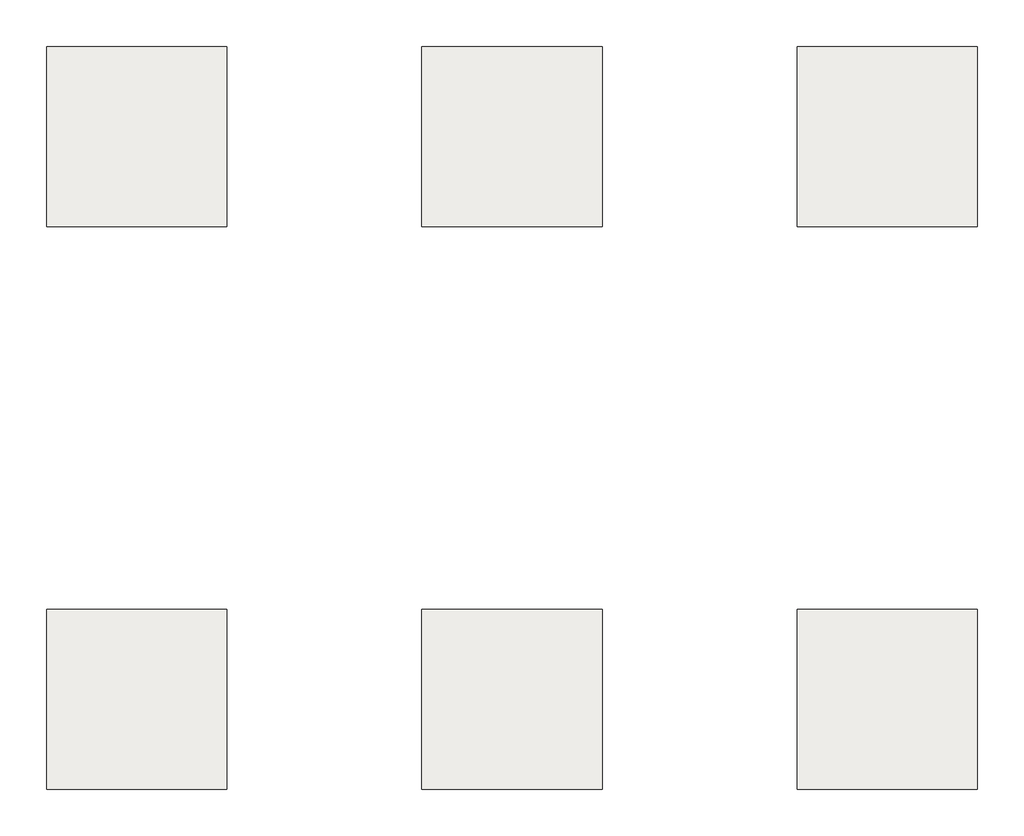
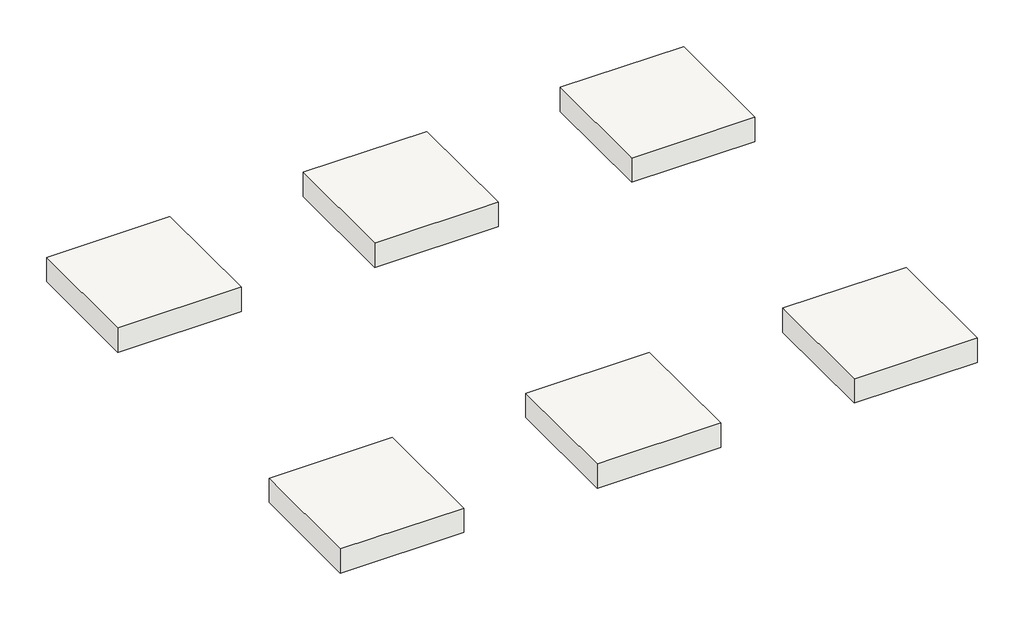
# Not in any storey: 6 slabs.
"""IFC4 building model written with IfcOpenShell, lengths in millimetres."""

import ifcopenshell
import ifcopenshell.guid

model = None  # the IFC model being written
_history = None  # IfcOwnerHistory: only IFC2X3 demands one
_inside = {}  # id of a spatial element -> (the spatial element, [elements in it])
_under = {}  # id of a project, library or spatial element -> (it, [spatial elements below it])
_declared = {}  # id of a project -> (the project, [libraries it declares])
_typed = {}  # id of a type object -> (the type object, [elements of that type])
_made_of = {}  # id of a material, layer set ... -> (it, [elements and type objects made of it])


def new_model(schema):
    """Start an empty IFC model of exactly this schema.

    Asked for "IFC4X3", IfcOpenShell would pick the latest addendum, in which some entities
    have other attributes; the version numbers below select the first issue.
    IFC2X3 requires an IfcOwnerHistory on every rooted entity: one is made here for all.
    """
    global model, _history
    if schema == "IFC4X3":
        model = ifcopenshell.file(schema_version=(4, 3, 0, 0))
    else:
        model = ifcopenshell.file(schema=schema)
    _inside.clear()
    _under.clear()
    _declared.clear()
    _typed.clear()
    _made_of.clear()
    _history = None
    if model.schema == "IFC2X3":
        org = make("IfcOrganization", Name="unknown")
        user = make(
            "IfcPersonAndOrganization",
            ThePerson=make("IfcPerson", FamilyName="unknown"),
            TheOrganization=org,
        )
        app = make(
            "IfcApplication",
            ApplicationDeveloper=org,
            Version="unknown",
            ApplicationFullName="unknown",
            ApplicationIdentifier="unknown",
        )
        _history = make(
            "IfcOwnerHistory",
            OwningUser=user,
            OwningApplication=app,
            ChangeAction="ADDED",
            CreationDate=0,
        )
    return model


def make(cls, **values):
    """One entity of the class cls with the attributes given. An attribute that is None is left unset."""
    return model.create_entity(
        cls, **{name: value for name, value in values.items() if value is not None}
    )


def rooted(cls, **values):
    """An entity with a GlobalId (a new one), such as an element, a storey or a relation."""
    return make(cls, GlobalId=ifcopenshell.guid.new(), OwnerHistory=_history, **values)


def si_unit(unit_type, name, prefix=None):
    """IfcSIUnit, for example si_unit("LENGTHUNIT", "METRE", prefix="MILLI")."""
    return make("IfcSIUnit", UnitType=unit_type, Prefix=prefix, Name=name)


def assignment(units):
    """IfcUnitAssignment: the units of a project."""
    return None if units is None else make("IfcUnitAssignment", Units=units)


def point(xyz):
    """IfcCartesianPoint."""
    return None if xyz is None else make("IfcCartesianPoint", Coordinates=xyz)


def direction(xyz):
    """IfcDirection."""
    return None if xyz is None else make("IfcDirection", DirectionRatios=xyz)


def frame(location, z_axis=None, x_axis=None):
    """IfcAxis2Placement3D, a coordinate frame: its origin and axes. An axis left out is left unset."""
    return make(
        "IfcAxis2Placement3D",
        Location=point(location),
        Axis=direction(z_axis),
        RefDirection=direction(x_axis),
    )


def origin():
    """The frame at (0, 0, 0) with its axes left unset."""
    return frame((0.0, 0.0, 0.0))


def place(relative_to, where):
    """IfcLocalPlacement: puts the frame where relative to a parent placement (None: the world)."""
    return make(
        "IfcLocalPlacement", PlacementRelTo=relative_to, RelativePlacement=where
    )


def context(
    kind, dimensions, precision=None, world=None, true_north=None, identifier=None
):
    """IfcGeometricRepresentationContext, for example the 3D "Model" context."""
    return make(
        "IfcGeometricRepresentationContext",
        ContextIdentifier=identifier,
        ContextType=kind,
        CoordinateSpaceDimension=dimensions,
        Precision=precision,
        WorldCoordinateSystem=world,
        TrueNorth=true_north,
    )


def project(units=None, contexts=None):
    """IfcProject with its units and contexts."""
    return rooted(
        "IfcProject",
        Name="project",
        RepresentationContexts=contexts,
        UnitsInContext=assignment(units),
    )


def spatial(cls, under=None, at=None, **own):
    """A site, building, storey or space (cls), placed at a placement, below another one or the project."""
    s = rooted(cls, ObjectPlacement=at, **own)
    if under is not None:
        _under.setdefault(under.id(), (under, []))[1].append(s)
    return s


def polyline(points):
    """IfcPolyline through the points."""
    return make("IfcPolyline", Points=[point(p) for p in points])


def outline(outer, holes=None, kind="AREA"):
    """IfcArbitraryClosedProfileDef: a profile drawn as a closed curve; with holes, ...WithVoids."""
    if holes is None:
        return make("IfcArbitraryClosedProfileDef", ProfileType=kind, OuterCurve=outer)
    return make(
        "IfcArbitraryProfileDefWithVoids",
        ProfileType=kind,
        OuterCurve=outer,
        InnerCurves=holes,
    )


def extrude(swept, where, along, depth):
    """IfcExtrudedAreaSolid: the profile swept, set in the frame where, extruded along a direction by depth."""
    return make(
        "IfcExtrudedAreaSolid",
        SweptArea=swept,
        Position=where,
        ExtrudedDirection=direction(along),
        Depth=depth,
    )


def shape(context_of_items, identifier, shape_type, items):
    """IfcShapeRepresentation: the items that make up one representation, for example the "Body"."""
    return make(
        "IfcShapeRepresentation",
        ContextOfItems=context_of_items,
        RepresentationIdentifier=identifier,
        RepresentationType=shape_type,
        Items=items,
    )


def source(mapping_origin, context_of_items, identifier, shape_type, items):
    """IfcRepresentationMap: a shape defined once, which mapped items show again and again."""
    return make(
        "IfcRepresentationMap",
        MappingOrigin=mapping_origin,
        MappedRepresentation=shape(context_of_items, identifier, shape_type, items),
    )


def transform(
    local_origin,
    x_axis=None,
    y_axis=None,
    z_axis=None,
    scale=None,
    scale2=None,
    scale3=None,
    uniform=True,
):
    """IfcCartesianTransformationOperator3D, or its non-uniform kind. x_axis, y_axis, z_axis: its Axis1, 2, 3."""
    if uniform:
        return make(
            "IfcCartesianTransformationOperator3D",
            Axis1=direction(x_axis),
            Axis2=direction(y_axis),
            LocalOrigin=point(local_origin),
            Scale=scale,
            Axis3=direction(z_axis),
        )
    return make(
        "IfcCartesianTransformationOperator3DnonUniform",
        Axis1=direction(x_axis),
        Axis2=direction(y_axis),
        LocalOrigin=point(local_origin),
        Scale=scale,
        Axis3=direction(z_axis),
        Scale2=scale2,
        Scale3=scale3,
    )


def mapped(mapping_source, mapping_target):
    """IfcMappedItem: shows the shape of a source again, moved by a transform."""
    return make(
        "IfcMappedItem", MappingSource=mapping_source, MappingTarget=mapping_target
    )


def made_of(thing, what):
    """Note that an element or type object is made of a material, layer set ...; save() writes the relation."""
    if what is not None:
        _made_of.setdefault(what.id(), (what, []))[1].append(thing)
    return thing


def element(
    cls,
    number,
    at=None,
    inside=None,
    cuts=None,
    type_object=None,
    material=None,
    context=None,
    identifier="Body",
    shape_type=None,
    held_by="IfcProductDefinitionShape",
    body=None,
    shapes=None,
    **own,
):
    """One element of the class cls, such as IfcWall. Its Tag is "e" and its number.

    at: its placement. inside: the storey or other place that contains it. cuts: it is an
    opening in that element (IfcRelVoidsElement). A single representation is given by context,
    identifier, shape_type and body (its items); several are given by shapes. held_by: the class
    of the entity that holds the representations. save() writes the other relations.
    """
    e = rooted(cls, Tag="e%d" % number, ObjectPlacement=at, **own)
    if body is not None:
        shapes = [shape(context, identifier, shape_type, body)]
    if shapes is not None:
        e.Representation = make(held_by, Representations=shapes)
    if inside is not None:
        _inside.setdefault(inside.id(), (inside, []))[1].append(e)
    if cuts is not None:
        rooted(
            "IfcRelVoidsElement", RelatingBuildingElement=cuts, RelatedOpeningElement=e
        )
    if type_object is not None:
        _typed.setdefault(type_object.id(), (type_object, []))[1].append(e)
    return made_of(e, material)


def aggregate(whole, parts):
    """IfcRelAggregates: a whole, such as a stair, and the parts it consists of."""
    return rooted("IfcRelAggregates", RelatingObject=whole, RelatedObjects=parts)


def save(model, path):
    """Write the relations noted so far, then the file.

    IfcRelAggregates (storeys below a building ...), IfcRelContainedInSpatialStructure (elements
    in a storey), IfcRelDefinesByType, IfcRelAssociatesMaterial and IfcRelDeclares: one each for
    every whole, place, type object, material and project.
    """
    for whole, parts in _under.values():
        aggregate(whole, parts)
    for where, things in _inside.values():
        rooted(
            "IfcRelContainedInSpatialStructure",
            RelatedElements=things,
            RelatingStructure=where,
        )
    for kind, things in _typed.values():
        rooted("IfcRelDefinesByType", RelatedObjects=things, RelatingType=kind)
    for what, things in _made_of.values():
        rooted("IfcRelAssociatesMaterial", RelatedObjects=things, RelatingMaterial=what)
    for by, libraries in _declared.values():
        rooted("IfcRelDeclares", RelatingContext=by, RelatedDefinitions=libraries)
    model.write(path)


def ft112_footing_rectangular_ft112_2400x2400x500_5fe39465(model_context):
    return source(origin(), model_context, "Body", "SweptSolid", [
        extrude(outline(polyline([(1200.0, 1200.0), (1200.0, -1200.0), (-1200.0, -1200.0), (-1200.0, 1200.0), (1200.0, 1200.0)])), frame((0.0, 0.0, -500.0), z_axis=(0.0, 0.0, 1.0), x_axis=(1.0, 0.0, 0.0)), (0.0, 0.0, 1.0), 500.0),
    ])


model = new_model("IFC4")

# Units and contexts
model_context = context("Model", 3, world=origin())
ifc_project = project(units=[si_unit("LENGTHUNIT", "METRE", prefix="MILLI")], contexts=[model_context])

# Site, building
site = spatial("IfcSite", under=ifc_project)
building = spatial("IfcBuilding", under=site)

# Slabs
placement = place(None, origin())
element("IfcSlab", 1, ObjectType="FT112-Footing-Rectangular : FT112_2400x2400x500", at=placement, inside=building, context=model_context, shape_type="SweptSolid", body=[
    extrude(outline(polyline([(11200.0, 22199.5208589), (11200.0, 19799.5208589), (8800.0, 19799.5208589), (8800.0, 22199.5208589), (11200.0, 22199.5208589)])), frame((0.0, 0.0, -1800.0), z_axis=(0.0, 0.0, 1.0), x_axis=(1.0, 0.0, 0.0)), (0.0, 0.0, 1.0), 500.0),
])
element("IfcSlab", 2, ObjectType="FT112-Footing-Rectangular : FT112_2400x2400x500", at=placement, inside=building, context=model_context, shape_type="SweptSolid", body=[
    extrude(outline(polyline([(6200.0, 22199.5208589), (6200.0, 19799.5208589), (3800.0, 19799.5208589), (3800.0, 22199.5208589), (6200.0, 22199.5208589)])), frame((0.0, 0.0, -1800.0), z_axis=(0.0, 0.0, 1.0), x_axis=(1.0, 0.0, 0.0)), (0.0, 0.0, 1.0), 500.0),
])
element("IfcSlab", 3, ObjectType="FT112-Footing-Rectangular : FT112_2400x2400x500", at=placement, inside=building, context=model_context, shape_type="SweptSolid", body=[
    extrude(outline(polyline([(1200.0, 22199.5208589), (1200.0, 19799.5208589), (-1200.0, 19799.5208589), (-1200.0, 22199.5208589), (1200.0, 22199.5208589)])), frame((0.0, 0.0, -1800.0), z_axis=(0.0, 0.0, 1.0), x_axis=(1.0, 0.0, 0.0)), (0.0, 0.0, 1.0), 500.0),
])
element("IfcSlab", 4, ObjectType="FT112-Footing-Rectangular : FT112_2400x2400x500", at=placement, inside=building, context=model_context, shape_type="SweptSolid", body=[
    extrude(outline(polyline([(1200.0, 14699.5208589), (1200.0, 12299.5208589), (-1200.0, 12299.5208589), (-1200.0, 14699.5208589), (1200.0, 14699.5208589)])), frame((0.0, 0.0, -1800.0), z_axis=(0.0, 0.0, 1.0), x_axis=(1.0, 0.0, 0.0)), (0.0, 0.0, 1.0), 500.0),
])
ft112_footing_rectangular_ft112_2400x2400x500_shape = ft112_footing_rectangular_ft112_2400x2400x500_5fe39465(model_context)
element("IfcSlab", 5, ObjectType="FT112-Footing-Rectangular : FT112_2400x2400x500", at=placement, inside=building, context=model_context, shape_type="MappedRepresentation", body=[
    mapped(ft112_footing_rectangular_ft112_2400x2400x500_shape, transform((5000.0, 13499.5208589, -1300.0), x_axis=(1.0, 0.0, 0.0), y_axis=(0.0, 1.0, 0.0), z_axis=(0.0, 0.0, 1.0))),
])
element("IfcSlab", 6, ObjectType="FT112-Footing-Rectangular : FT112_2400x2400x500", at=placement, inside=building, context=model_context, shape_type="MappedRepresentation", body=[
    mapped(ft112_footing_rectangular_ft112_2400x2400x500_shape, transform((10000.0, 13499.5208589, -1300.0), x_axis=(1.0, 0.0, 0.0), y_axis=(0.0, 1.0, 0.0), z_axis=(0.0, 0.0, 1.0))),
])

save(model, "model.ifc")

# Revit data of these elements
# Project information
#   Building Name = "MAIN GATE SECURITY BUILDING"
#   Project Status = "Project Status"
#   Client Name = "현대엔지니어링"
#   Project Address = "서울시 종로구 율곡로 75(계동)"
#   Project Name = "Therma Visayas Energy Project"
#   Project Number = "-"
# Grids (mm)
#   "A": line (0, 24502.793) -> (0, 11308.625)
#   "B": line (5000, 24502.793) -> (5000, 11308.625)
#   "C": line (10000, 24502.793) -> (10000, 11308.625)
#   "1": line (-3860.098, 13499.521) -> (12441.468, 13499.521)
#   "2": line (-3860.098, 20999.521) -> (12441.468, 20999.521)
# Type "FT112-Footing-Rectangular : FT112_2400x2400x500"
#   Type Mark = "A"
#   Top bar = ""
#   Description = "UG Shallow Foundation"
#   Bottom bar = "D20@300"
#   Width = 2400 mm
#   Length = 2400 mm
#   Foundation Thickness = 500 mm
#   hec_material3 [instance default] = none
#   hec_material2 [instance default] = A03AE056-00001_Bitumen/Bituminous/Asphalt Coating
#   hec_material1 [instance default] = A03AC035-00001_Form Work (3 times in use)_Flat
#   Structural Material [instance default] = A03AC032-00007_Structural Concrete_Type1_25MPa-30Mpa
#   Assembly Code = ""
# Elements 1, 2, 3, 4, 5, 6 (IfcSlab, "FT112-Footing-Rectangular : FT112_2400x2400x500")
#   Comments = ""
#   Mark = "F1"
#   F01) Building Name = "Main Gate House"
#   F11) Project Building Tag_Type-1 = "Common"
#   F12) Project Building Tag_Type-2 = "Common"
#   F13) Project Facility Code = "Facility Code"
#   F21) Structural Type = "Concrete"
#   F31) Standard Building Code = "IBC"
#   F41) Discipline = "AR"
#   F51) Plan Start Date-Engineering = "2015-01-01"
#   F52) Plan Finish Date-Engineering = "2015-12-31"
#   F53) Duration = "365"
#   F54) Actual Start Date-Engineering = "2015-01-01"
#   F55) Actual Finish Date-Engineering = "2015-12-31"
#   F61) Plan Start Date-Construction = "2016-08-19"
#   F62) Plan Finish Date-Construction = "2017-01-31"
#   F64) Actual Start Date-Construction = "2016-08-19"
#   F63) Duration = "202"
#   F65) Actual Finish Date-Construction = "2017-01-31"
#   F91) Plant Type = "CFPP"
#   F92) KKS Structures, Building = "UYF"
#   P01) Project Name = "TVEP"
#   P02) Project Configuration = "CFB Boiler x 2(Foster Wheeler) + STG x 2(Alstom, 150MW)"
#   P03) Project Abbreviation = "TVEP"
#   P04) Project Code = "BEPH1402"
#   P05) Project Stage = "In operation"
#   P06) Project Location = "Sito Looc, Barangay Bato, Toledo City in Philippines"
#   P07) Project Owner = "Therma Visayas, Inc."
#   P08) Project O.E = "Flour"
#   P09) Project Schedule = "ITB Issueing Date : 2013.07.30\r\nSite Survey : 2013.08.19-20\r\nBid Closing Date : 2013.11.29\r\nPreferred Bidder Notice 접수 : 2014.04.27\r\nTarget award date : 2014 05\r\nLOA 접수 : 2014.05.21\r\nSigning Ceremony : 2014.05.30"
#   P10) Basic Wind Speed = "55.6 m/s"
#   P11) Seismic = "NSCP 2010, Zone 4 (PGA : 0.4g)"
#   P12) Soil = "Sc"
#   P13) Soil Capacity = "100kN/m2"
#   P14) Pile Capacity = "PHC(D400) : 1200kN"
#   W00) Work Master Code = "A03AC032-00007"
#   W01) Work Master_Lv1 = "Concrete Work"
#   W02) Work Master_Lv2 = "Substructure Work"
#   W03) Work Master_Spec.1 = "Cement Type-1"
#   W04) Work Master_Spec.2 = "25MPa < F'c (Cylinder Strength) ≤ 30MPa"
#   W11) Activity ID = "C02AGB010"
#   W12) Activity Name = "Main Gate Security Building - Building Foundation"
#   W13) Plan Start Date = "2016-08-19"
#   W14) Plan Finish Date = "2016-09-22"
#   W15) Duration = "26"
#   W16) Actual Start Date = "2016-08-19"
#   W17) Actual Finish Date = "2016-09-22"
#   TOP BAR = "D22 @250"
#   BOTTOM BAR = "D12 @250"
#   R02) Unit Price = 0
#   Structural Material = A03AD032-00007_Structural Concrete_25MPa-30MPa
#   hec_material3 = none
#   hec_material2 = none
#   hec_material1 = none
#   Phase Created = New Construction
#   Materials on its faces: "A03AD032-00007_Structural Concrete_25MPa-30MPa"
# Materials
#   "A03AE056-00001_Bitumen/Bituminous/Asphalt Coating": class "Generic", colour RGB 17 17 17, transparency 0, Description = "Damp-proofing", W00) Work Master Code = "A03AE056-00001", W01) Work Master_Lv1 = "Concrete Work", W02) Work Master_Lv2 = "Concrete Protective Coating (U/G)", W03) Work Master_Spec.1 = "Bitumen/Bituminous/Asphalt Coating", Cost = 0
#   "A03AC035-00001_Form Work (3 times in use)_Flat": class "Wood", colour RGB 149 120 74, transparency 0, Description = "Plywood", W00) Work Master Code = "A03AC035-00001", W01) Work Master_Lv1 = "Concrete Work", W02) Work Master_Lv2 = "Substructure Work", W03) Work Master_Spec.1 = "Form Work (3 times in use)", W04) Work Master_Spec.2 = "Flat Form", W05) Work Master_Spec.3 = "Dressed Lumber, Plywood or Steel Form(Wood Planks are not Allowed) incl. Chamfer", Cost = 0
#   "A03AC032-00007_Structural Concrete_Type1_25MPa-30Mpa": class "Concrete", colour RGB 176 176 176, transparency 0, Keynote = "09910.A1", Description = "Reinf. Conc.", W00) Work Master Code = "A03AC032-00007", W01) Work Master_Lv1 = "Concrete Work", W02) Work Master_Lv2 = "Substructure Work", W03) Work Master_Spec.1 = "Structural Concrete", W04) Work Master_Spec.2 = "Cement Type-1", W05) Work Master_Spec.3 = "25MPa < F'c (Cylinder Strength) ≤ 30MPa", Cost = 0
#   "A03AD032-00007_Structural Concrete_25MPa-30MPa": class "Concrete", colour RGB 176 176 176, transparency 0, Keynote = "09910.A1", Description = "LATEX PAINT ON F.F CONC.", W00) Work Master Code = "A03AD032-00007", W01) Work Master_Lv1 = "Concrete Work", W02) Work Master_Lv2 = "Superstructure Work", W03) Work Master_Spec.1 = "Structural Concrete", W04) Work Master_Spec.2 = "Cement Type-1", W05) Work Master_Spec.3 = "25MPa < F'c (Cylinder Strength) ≤ 30MPa", Cost = 0
